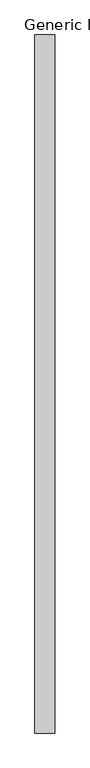
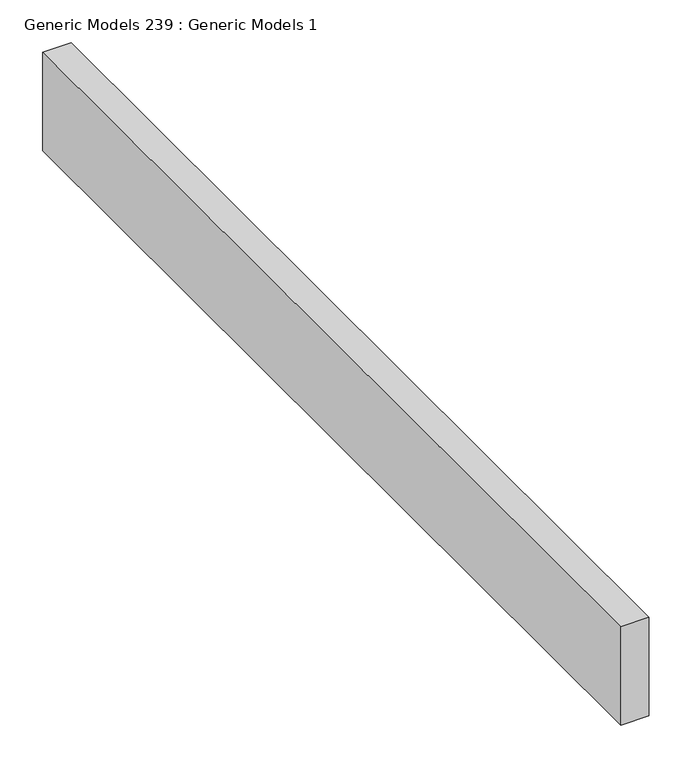
"""IFC4 building model written with IfcOpenShell, lengths in millimetres: proxy geometry, Generic Models 239 : Generic Models 1."""

from ifc_helpers import new_model, si_unit, frame, origin, place, context, project, spatial, polyline, outline, extrude, source, transform, mapped, element, save


def generic_models_239_generic_models_1_18037994(model_context):
    return source(origin(), model_context, "Body", "SweptSolid", [
        extrude(outline(polyline([(1003.1263704, 10554.2870839), (965.0263704, 10554.2870839), (965.0263704, 11900.4870839), (1003.1263704, 11900.4870839), (1003.1263704, 10554.2870839)])), frame((0.0, 0.0, 126383.796), z_axis=(0.0, 0.0, 1.0), x_axis=(1.0, 0.0, 0.0)), (0.0, 0.0, 1.0), 139.7),
    ])


if __name__ == "__main__":
    model = new_model("IFC4")
    model_context = context("Model", 3, world=origin())
    ifc_project = project(units=[si_unit("LENGTHUNIT", "METRE", prefix="MILLI")], contexts=[model_context])
    site = spatial("IfcSite", under=ifc_project)
    building = spatial("IfcBuilding", under=site)
    placement = place(None, origin())
    generic_models_239_generic_models_1_shape = generic_models_239_generic_models_1_18037994(model_context)
    element("IfcBuildingElementProxy", 1, Name="Generic Models 239 : Generic Models 1", ObjectType="Generic Models 239 : Generic Models 1", at=placement, inside=building, context=model_context, shape_type="MappedRepresentation", body=[
        mapped(generic_models_239_generic_models_1_shape, transform((0.0, 0.0, 0.0), x_axis=(1.0, 0.0, 0.0), y_axis=(0.0, 1.0, 0.0), z_axis=(0.0, 0.0, 1.0))),
    ])
    save(model, "model.ifc")

# Revit data of these elements
# Element 1 (IfcBuildingElementProxy, "Generic Models 239 : Generic Models 1")
#   Materials on its faces: "_STRUCTURAL MEMBER (SEE STRUCT. DWGS)"
# Materials
#   "_STRUCTURAL MEMBER (SEE STRUCT. DWGS)": class "Generic", colour RGB 209 182 141, transparency 0, Cost = 0
